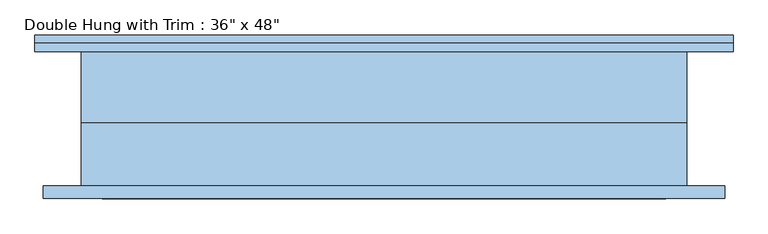
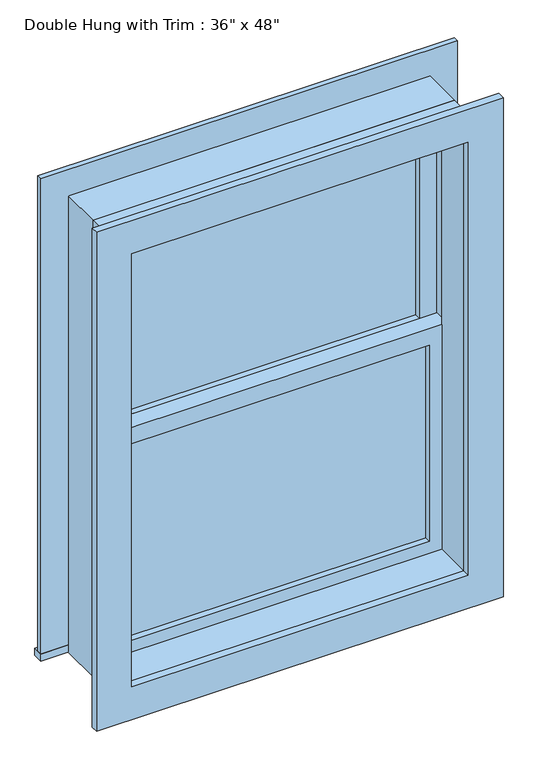
"""IFC4 building model written with IfcOpenShell, lengths in millimetres: window geometry."""

import ifcopenshell
import ifcopenshell.guid

model = None  # the IFC model being written
_history = None  # IfcOwnerHistory: only IFC2X3 demands one
_inside = {}  # id of a spatial element -> (the spatial element, [elements in it])
_under = {}  # id of a project, library or spatial element -> (it, [spatial elements below it])
_declared = {}  # id of a project -> (the project, [libraries it declares])
_typed = {}  # id of a type object -> (the type object, [elements of that type])
_made_of = {}  # id of a material, layer set ... -> (it, [elements and type objects made of it])


def new_model(schema):
    """Start an empty IFC model of exactly this schema.

    Asked for "IFC4X3", IfcOpenShell would pick the latest addendum, in which some entities
    have other attributes; the version numbers below select the first issue.
    IFC2X3 requires an IfcOwnerHistory on every rooted entity: one is made here for all.
    """
    global model, _history
    if schema == "IFC4X3":
        model = ifcopenshell.file(schema_version=(4, 3, 0, 0))
    else:
        model = ifcopenshell.file(schema=schema)
    _inside.clear()
    _under.clear()
    _declared.clear()
    _typed.clear()
    _made_of.clear()
    _history = None
    if model.schema == "IFC2X3":
        org = make("IfcOrganization", Name="unknown")
        user = make(
            "IfcPersonAndOrganization",
            ThePerson=make("IfcPerson", FamilyName="unknown"),
            TheOrganization=org,
        )
        app = make(
            "IfcApplication",
            ApplicationDeveloper=org,
            Version="unknown",
            ApplicationFullName="unknown",
            ApplicationIdentifier="unknown",
        )
        _history = make(
            "IfcOwnerHistory",
            OwningUser=user,
            OwningApplication=app,
            ChangeAction="ADDED",
            CreationDate=0,
        )
    return model


def make(cls, **values):
    """One entity of the class cls with the attributes given. An attribute that is None is left unset."""
    return model.create_entity(
        cls, **{name: value for name, value in values.items() if value is not None}
    )


def rooted(cls, **values):
    """An entity with a GlobalId (a new one), such as an element, a storey or a relation."""
    return make(cls, GlobalId=ifcopenshell.guid.new(), OwnerHistory=_history, **values)


def si_unit(unit_type, name, prefix=None):
    """IfcSIUnit, for example si_unit("LENGTHUNIT", "METRE", prefix="MILLI")."""
    return make("IfcSIUnit", UnitType=unit_type, Prefix=prefix, Name=name)


def assignment(units):
    """IfcUnitAssignment: the units of a project."""
    return None if units is None else make("IfcUnitAssignment", Units=units)


def point(xyz):
    """IfcCartesianPoint."""
    return None if xyz is None else make("IfcCartesianPoint", Coordinates=xyz)


def direction(xyz):
    """IfcDirection."""
    return None if xyz is None else make("IfcDirection", DirectionRatios=xyz)


def frame(location, z_axis=None, x_axis=None):
    """IfcAxis2Placement3D, a coordinate frame: its origin and axes. An axis left out is left unset."""
    return make(
        "IfcAxis2Placement3D",
        Location=point(location),
        Axis=direction(z_axis),
        RefDirection=direction(x_axis),
    )


def origin():
    """The frame at (0, 0, 0) with its axes left unset."""
    return frame((0.0, 0.0, 0.0))


def place(relative_to, where):
    """IfcLocalPlacement: puts the frame where relative to a parent placement (None: the world)."""
    return make(
        "IfcLocalPlacement", PlacementRelTo=relative_to, RelativePlacement=where
    )


def context(
    kind, dimensions, precision=None, world=None, true_north=None, identifier=None
):
    """IfcGeometricRepresentationContext, for example the 3D "Model" context."""
    return make(
        "IfcGeometricRepresentationContext",
        ContextIdentifier=identifier,
        ContextType=kind,
        CoordinateSpaceDimension=dimensions,
        Precision=precision,
        WorldCoordinateSystem=world,
        TrueNorth=true_north,
    )


def project(units=None, contexts=None):
    """IfcProject with its units and contexts."""
    return rooted(
        "IfcProject",
        Name="project",
        RepresentationContexts=contexts,
        UnitsInContext=assignment(units),
    )


def spatial(cls, under=None, at=None, **own):
    """A site, building, storey or space (cls), placed at a placement, below another one or the project."""
    s = rooted(cls, ObjectPlacement=at, **own)
    if under is not None:
        _under.setdefault(under.id(), (under, []))[1].append(s)
    return s


def polyline(points):
    """IfcPolyline through the points."""
    return make("IfcPolyline", Points=[point(p) for p in points])


def outline(outer, holes=None, kind="AREA"):
    """IfcArbitraryClosedProfileDef: a profile drawn as a closed curve; with holes, ...WithVoids."""
    if holes is None:
        return make("IfcArbitraryClosedProfileDef", ProfileType=kind, OuterCurve=outer)
    return make(
        "IfcArbitraryProfileDefWithVoids",
        ProfileType=kind,
        OuterCurve=outer,
        InnerCurves=holes,
    )


def extrude(swept, where, along, depth):
    """IfcExtrudedAreaSolid: the profile swept, set in the frame where, extruded along a direction by depth."""
    return make(
        "IfcExtrudedAreaSolid",
        SweptArea=swept,
        Position=where,
        ExtrudedDirection=direction(along),
        Depth=depth,
    )


def shape(context_of_items, identifier, shape_type, items):
    """IfcShapeRepresentation: the items that make up one representation, for example the "Body"."""
    return make(
        "IfcShapeRepresentation",
        ContextOfItems=context_of_items,
        RepresentationIdentifier=identifier,
        RepresentationType=shape_type,
        Items=items,
    )


def source(mapping_origin, context_of_items, identifier, shape_type, items):
    """IfcRepresentationMap: a shape defined once, which mapped items show again and again."""
    return make(
        "IfcRepresentationMap",
        MappingOrigin=mapping_origin,
        MappedRepresentation=shape(context_of_items, identifier, shape_type, items),
    )


def transform(
    local_origin,
    x_axis=None,
    y_axis=None,
    z_axis=None,
    scale=None,
    scale2=None,
    scale3=None,
    uniform=True,
):
    """IfcCartesianTransformationOperator3D, or its non-uniform kind. x_axis, y_axis, z_axis: its Axis1, 2, 3."""
    if uniform:
        return make(
            "IfcCartesianTransformationOperator3D",
            Axis1=direction(x_axis),
            Axis2=direction(y_axis),
            LocalOrigin=point(local_origin),
            Scale=scale,
            Axis3=direction(z_axis),
        )
    return make(
        "IfcCartesianTransformationOperator3DnonUniform",
        Axis1=direction(x_axis),
        Axis2=direction(y_axis),
        LocalOrigin=point(local_origin),
        Scale=scale,
        Axis3=direction(z_axis),
        Scale2=scale2,
        Scale3=scale3,
    )


def mapped(mapping_source, mapping_target):
    """IfcMappedItem: shows the shape of a source again, moved by a transform."""
    return make(
        "IfcMappedItem", MappingSource=mapping_source, MappingTarget=mapping_target
    )


def made_of(thing, what):
    """Note that an element or type object is made of a material, layer set ...; save() writes the relation."""
    if what is not None:
        _made_of.setdefault(what.id(), (what, []))[1].append(thing)
    return thing


def element(
    cls,
    number,
    at=None,
    inside=None,
    cuts=None,
    type_object=None,
    material=None,
    context=None,
    identifier="Body",
    shape_type=None,
    held_by="IfcProductDefinitionShape",
    body=None,
    shapes=None,
    **own,
):
    """One element of the class cls, such as IfcWall. Its Tag is "e" and its number.

    at: its placement. inside: the storey or other place that contains it. cuts: it is an
    opening in that element (IfcRelVoidsElement). A single representation is given by context,
    identifier, shape_type and body (its items); several are given by shapes. held_by: the class
    of the entity that holds the representations. save() writes the other relations.
    """
    e = rooted(cls, Tag="e%d" % number, ObjectPlacement=at, **own)
    if body is not None:
        shapes = [shape(context, identifier, shape_type, body)]
    if shapes is not None:
        e.Representation = make(held_by, Representations=shapes)
    if inside is not None:
        _inside.setdefault(inside.id(), (inside, []))[1].append(e)
    if cuts is not None:
        rooted(
            "IfcRelVoidsElement", RelatingBuildingElement=cuts, RelatedOpeningElement=e
        )
    if type_object is not None:
        _typed.setdefault(type_object.id(), (type_object, []))[1].append(e)
    return made_of(e, material)


def aggregate(whole, parts):
    """IfcRelAggregates: a whole, such as a stair, and the parts it consists of."""
    return rooted("IfcRelAggregates", RelatingObject=whole, RelatedObjects=parts)


def save(model, path):
    """Write the relations noted so far, then the file.

    IfcRelAggregates (storeys below a building ...), IfcRelContainedInSpatialStructure (elements
    in a storey), IfcRelDefinesByType, IfcRelAssociatesMaterial and IfcRelDeclares: one each for
    every whole, place, type object, material and project.
    """
    for whole, parts in _under.values():
        aggregate(whole, parts)
    for where, things in _inside.values():
        rooted(
            "IfcRelContainedInSpatialStructure",
            RelatedElements=things,
            RelatingStructure=where,
        )
    for kind, things in _typed.values():
        rooted("IfcRelDefinesByType", RelatedObjects=things, RelatingType=kind)
    for what, things in _made_of.values():
        rooted("IfcRelAssociatesMaterial", RelatedObjects=things, RelatingMaterial=what)
    for by, libraries in _declared.values():
        rooted("IfcRelDeclares", RelatingContext=by, RelatedDefinitions=libraries)
    model.write(path)


def window_31198920(model_context):
    return source(origin(), model_context, "Body", "SweptSolid", [
        extrude(outline(polyline([(-393.7, 22.225), (393.7, 22.225), (393.7, 9.525), (-393.7, 9.525), (-393.7, 22.225)])), frame((0.0, 0.0, 977.9), z_axis=(0.0, 0.0, 1.0), x_axis=(1.0, 0.0, 0.0)), (0.0, 0.0, 1.0), 523.875),
        extrude(outline(polyline([(1546.225, -438.15), (933.45, -438.15), (933.45, 438.15), (1546.225, 438.15), (1546.225, -438.15)]), holes=[polyline([(1501.775, -393.7), (1501.775, 393.7), (977.9, 393.7), (977.9, -393.7), (1501.775, -393.7)])]), frame((0.0, -6.35, 0.0), z_axis=(0.0, 1.0, 0.0), x_axis=(0.0, 0.0, 1.0)), (0.0, 0.0, 1.0), 44.45),
        extrude(outline(polyline([(-527.05, 127.0), (527.05, 127.0), (527.05, 101.6), (-527.05, 101.6), (-527.05, 127.0)])), frame((0.0, 0.0, 914.4), z_axis=(0.0, 0.0, 1.0), x_axis=(1.0, 0.0, 0.0)), (0.0, 0.0, 1.0), 19.05),
        extrude(outline(polyline([(2114.55, -438.15), (2114.55, 438.15), (933.45, 438.15), (933.45, 527.05), (2203.45, 527.05), (2203.45, -527.05), (933.45, -527.05), (933.45, -438.15), (2114.55, -438.15)])), frame((0.0, 101.6, 0.0), z_axis=(0.0, 1.0, 0.0), x_axis=(0.0, 0.0, 1.0)), (0.0, 0.0, 1.0), 12.7),
        extrude(outline(polyline([(2190.75, 514.35), (2190.75, -514.35), (857.25, -514.35), (857.25, 514.35), (2190.75, 514.35)]), holes=[polyline([(2101.85, 425.45), (946.15, 425.45), (946.15, -425.45), (2101.85, -425.45), (2101.85, 425.45)])]), frame((0.0, -120.65, 0.0), z_axis=(0.0, 1.0, 0.0), x_axis=(0.0, 0.0, 1.0)), (0.0, 0.0, 1.0), 19.05),
        extrude(outline(polyline([(393.7, 53.975), (-393.7, 53.975), (-393.7, 66.675), (393.7, 66.675), (393.7, 53.975)])), frame((0.0, 0.0, 1546.225), z_axis=(0.0, 0.0, 1.0), x_axis=(1.0, 0.0, 0.0)), (0.0, 0.0, 1.0), 523.875),
        extrude(outline(polyline([(2114.55, -438.15), (1501.775, -438.15), (1501.775, 438.15), (2114.55, 438.15), (2114.55, -438.15)]), holes=[polyline([(2070.1, -393.7), (2070.1, 393.7), (1546.225, 393.7), (1546.225, -393.7), (2070.1, -393.7)])]), frame((0.0, 38.1, 0.0), z_axis=(0.0, 1.0, 0.0), x_axis=(0.0, 0.0, 1.0)), (0.0, 0.0, 1.0), 44.45),
        extrude(outline(polyline([(2133.6, -457.2), (914.4, -457.2), (914.4, 457.2), (2133.6, 457.2), (2133.6, -457.2)]), holes=[polyline([(2101.85, -425.45), (2101.85, 425.45), (946.15, 425.45), (946.15, -425.45), (2101.85, -425.45)])]), frame((0.0, -101.6, 0.0), z_axis=(0.0, 1.0, 0.0), x_axis=(0.0, 0.0, 1.0)), (0.0, 0.0, 1.0), 95.25),
        extrude(outline(polyline([(2133.6, 457.2), (2133.6, -457.2), (914.4, -457.2), (914.4, 457.2), (2133.6, 457.2)]), holes=[polyline([(2114.55, 438.15), (933.45, 438.15), (933.45, -438.15), (2114.55, -438.15), (2114.55, 438.15)])]), frame((0.0, -6.35, 0.0), z_axis=(0.0, 1.0, 0.0), x_axis=(0.0, 0.0, 1.0)), (0.0, 0.0, 1.0), 107.95),
    ])


if __name__ == "__main__":
    model = new_model("IFC4")
    model_context = context("Model", 3, world=origin())
    ifc_project = project(units=[si_unit("LENGTHUNIT", "METRE", prefix="MILLI")], contexts=[model_context])
    site = spatial("IfcSite", under=ifc_project)
    building = spatial("IfcBuilding", under=site)
    placement = place(None, origin())
    window_shape = window_31198920(model_context)
    element("IfcWindow", 1, ObjectType="Double Hung with Trim : 36\" x 48\"", at=placement, inside=building, context=model_context, shape_type="MappedRepresentation", body=[
        mapped(window_shape, transform((0.0, 0.0, 0.0), x_axis=(1.0, 0.0, 0.0), y_axis=(0.0, 1.0, 0.0), z_axis=(0.0, 0.0, 1.0))),
    ])
    save(model, "model.ifc")

# Revit data of these elements
# Type "Double Hung with Trim : 36\" x 48\""
#   Type Mark = "13"
#   Construction Type Id = "GSP4R"
#   Assembly Code = "B2020100"
#   Analytic Construction = "1/8 in Pilkington single glazing"
#   Visual Light Transmittance = 0.9
#   Solar Heat Gain Coefficient = 0.78
#   Heat Transfer Coefficient (U) = 3.6886 W/(m²·K)
#   Height = 4' - 0"
#   Default Sill Height = 3' - 0"
#   Trim Projection - Ext. = 0' - 0 1/2"
#   Trim Projection - Int. = 0' - 0 3/4"
#   Trim Width - Exterior = 0' - 3 1/2"
#   Trim Width - Interior = 0' - 3 1/2"
#   Width = 3' - 0"
#   Window Inset = 0' - 0 3/4"
#   Glass Pane Material = Glass
#   Sash Material = Sash
#   Trim Exterior Material = Trim
#   Trim Interior Material = Trim
#   Wall Closure = (empty or 0)
# Element 1 (IfcWindow, "Double Hung with Trim : 36\" x 48\"")
#   Materials on its faces: "Sash", "Trim", "Glass"
# Materials
#   "Glass": class "Glass", colour RGB 0 128 192, transparency 0.75, Description = "Soda Lime Glass", Cost = 0
#   "Sash": class "Wood", colour RGB 224 178 126, transparency 0, Cost = 0
#   "Trim": class "Wood", colour RGB 224 178 126, transparency 0
